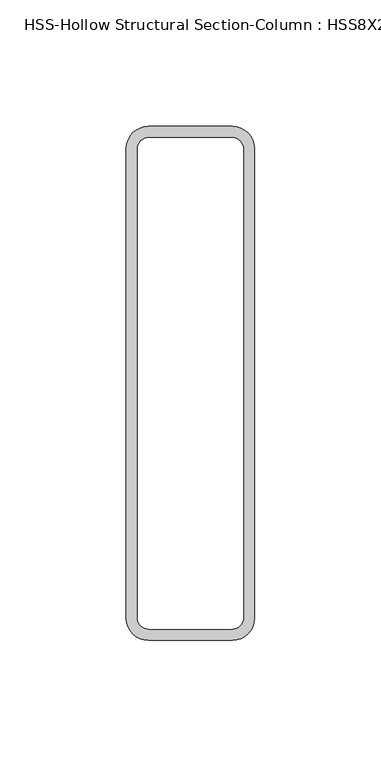
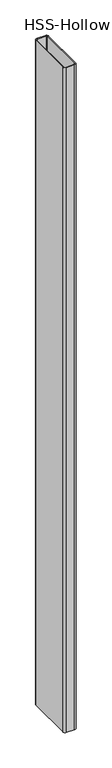
"""IFC4 building model written with IfcOpenShell, lengths in millimetres: column geometry, HSS-Hollow Structural Section-Column : HSS8X2X3/16."""

import ifcopenshell
import ifcopenshell.guid

model = None  # the IFC model being written
_history = None  # IfcOwnerHistory: only IFC2X3 demands one
_inside = {}  # id of a spatial element -> (the spatial element, [elements in it])
_under = {}  # id of a project, library or spatial element -> (it, [spatial elements below it])
_declared = {}  # id of a project -> (the project, [libraries it declares])
_typed = {}  # id of a type object -> (the type object, [elements of that type])
_made_of = {}  # id of a material, layer set ... -> (it, [elements and type objects made of it])


def new_model(schema):
    """Start an empty IFC model of exactly this schema.

    Asked for "IFC4X3", IfcOpenShell would pick the latest addendum, in which some entities
    have other attributes; the version numbers below select the first issue.
    IFC2X3 requires an IfcOwnerHistory on every rooted entity: one is made here for all.
    """
    global model, _history
    if schema == "IFC4X3":
        model = ifcopenshell.file(schema_version=(4, 3, 0, 0))
    else:
        model = ifcopenshell.file(schema=schema)
    _inside.clear()
    _under.clear()
    _declared.clear()
    _typed.clear()
    _made_of.clear()
    _history = None
    if model.schema == "IFC2X3":
        org = make("IfcOrganization", Name="unknown")
        user = make(
            "IfcPersonAndOrganization",
            ThePerson=make("IfcPerson", FamilyName="unknown"),
            TheOrganization=org,
        )
        app = make(
            "IfcApplication",
            ApplicationDeveloper=org,
            Version="unknown",
            ApplicationFullName="unknown",
            ApplicationIdentifier="unknown",
        )
        _history = make(
            "IfcOwnerHistory",
            OwningUser=user,
            OwningApplication=app,
            ChangeAction="ADDED",
            CreationDate=0,
        )
    return model


def make(cls, **values):
    """One entity of the class cls with the attributes given. An attribute that is None is left unset."""
    return model.create_entity(
        cls, **{name: value for name, value in values.items() if value is not None}
    )


def rooted(cls, **values):
    """An entity with a GlobalId (a new one), such as an element, a storey or a relation."""
    return make(cls, GlobalId=ifcopenshell.guid.new(), OwnerHistory=_history, **values)


def si_unit(unit_type, name, prefix=None):
    """IfcSIUnit, for example si_unit("LENGTHUNIT", "METRE", prefix="MILLI")."""
    return make("IfcSIUnit", UnitType=unit_type, Prefix=prefix, Name=name)


def assignment(units):
    """IfcUnitAssignment: the units of a project."""
    return None if units is None else make("IfcUnitAssignment", Units=units)


def point(xyz):
    """IfcCartesianPoint."""
    return None if xyz is None else make("IfcCartesianPoint", Coordinates=xyz)


def direction(xyz):
    """IfcDirection."""
    return None if xyz is None else make("IfcDirection", DirectionRatios=xyz)


def frame(location, z_axis=None, x_axis=None):
    """IfcAxis2Placement3D, a coordinate frame: its origin and axes. An axis left out is left unset."""
    return make(
        "IfcAxis2Placement3D",
        Location=point(location),
        Axis=direction(z_axis),
        RefDirection=direction(x_axis),
    )


def frame_2d(location, x_axis=None):
    """IfcAxis2Placement2D, a coordinate frame in the plane: its origin and x axis."""
    return make(
        "IfcAxis2Placement2D", Location=point(location), RefDirection=direction(x_axis)
    )


def origin():
    """The frame at (0, 0, 0) with its axes left unset."""
    return frame((0.0, 0.0, 0.0))


def place(relative_to, where):
    """IfcLocalPlacement: puts the frame where relative to a parent placement (None: the world)."""
    return make(
        "IfcLocalPlacement", PlacementRelTo=relative_to, RelativePlacement=where
    )


def context(
    kind, dimensions, precision=None, world=None, true_north=None, identifier=None
):
    """IfcGeometricRepresentationContext, for example the 3D "Model" context."""
    return make(
        "IfcGeometricRepresentationContext",
        ContextIdentifier=identifier,
        ContextType=kind,
        CoordinateSpaceDimension=dimensions,
        Precision=precision,
        WorldCoordinateSystem=world,
        TrueNorth=true_north,
    )


def project(units=None, contexts=None):
    """IfcProject with its units and contexts."""
    return rooted(
        "IfcProject",
        Name="project",
        RepresentationContexts=contexts,
        UnitsInContext=assignment(units),
    )


def spatial(cls, under=None, at=None, **own):
    """A site, building, storey or space (cls), placed at a placement, below another one or the project."""
    s = rooted(cls, ObjectPlacement=at, **own)
    if under is not None:
        _under.setdefault(under.id(), (under, []))[1].append(s)
    return s


def polyline(points):
    """IfcPolyline through the points."""
    return make("IfcPolyline", Points=[point(p) for p in points])


def circle_curve(where, radius):
    """IfcCircle in the frame where."""
    return make("IfcCircle", Position=where, Radius=radius)


def trimmed(basis, trim1, trim2, sense, master):
    """IfcTrimmedCurve: the piece of a basis curve between two trims."""
    return make(
        "IfcTrimmedCurve",
        BasisCurve=basis,
        Trim1=trim1,
        Trim2=trim2,
        SenseAgreement=sense,
        MasterRepresentation=master,
    )


def segment(curve, same_sense, transition):
    """IfcCompositeCurveSegment."""
    return make(
        "IfcCompositeCurveSegment",
        Transition=transition,
        SameSense=same_sense,
        ParentCurve=curve,
    )


def composite_curve(segments, self_intersect=None):
    """IfcCompositeCurve: segments joined end to end."""
    return make("IfcCompositeCurve", Segments=segments, SelfIntersect=self_intersect)


def outline(outer, holes=None, kind="AREA"):
    """IfcArbitraryClosedProfileDef: a profile drawn as a closed curve; with holes, ...WithVoids."""
    if holes is None:
        return make("IfcArbitraryClosedProfileDef", ProfileType=kind, OuterCurve=outer)
    return make(
        "IfcArbitraryProfileDefWithVoids",
        ProfileType=kind,
        OuterCurve=outer,
        InnerCurves=holes,
    )


def extrude(swept, where, along, depth):
    """IfcExtrudedAreaSolid: the profile swept, set in the frame where, extruded along a direction by depth."""
    return make(
        "IfcExtrudedAreaSolid",
        SweptArea=swept,
        Position=where,
        ExtrudedDirection=direction(along),
        Depth=depth,
    )


def shape(context_of_items, identifier, shape_type, items):
    """IfcShapeRepresentation: the items that make up one representation, for example the "Body"."""
    return make(
        "IfcShapeRepresentation",
        ContextOfItems=context_of_items,
        RepresentationIdentifier=identifier,
        RepresentationType=shape_type,
        Items=items,
    )


def source(mapping_origin, context_of_items, identifier, shape_type, items):
    """IfcRepresentationMap: a shape defined once, which mapped items show again and again."""
    return make(
        "IfcRepresentationMap",
        MappingOrigin=mapping_origin,
        MappedRepresentation=shape(context_of_items, identifier, shape_type, items),
    )


def transform(
    local_origin,
    x_axis=None,
    y_axis=None,
    z_axis=None,
    scale=None,
    scale2=None,
    scale3=None,
    uniform=True,
):
    """IfcCartesianTransformationOperator3D, or its non-uniform kind. x_axis, y_axis, z_axis: its Axis1, 2, 3."""
    if uniform:
        return make(
            "IfcCartesianTransformationOperator3D",
            Axis1=direction(x_axis),
            Axis2=direction(y_axis),
            LocalOrigin=point(local_origin),
            Scale=scale,
            Axis3=direction(z_axis),
        )
    return make(
        "IfcCartesianTransformationOperator3DnonUniform",
        Axis1=direction(x_axis),
        Axis2=direction(y_axis),
        LocalOrigin=point(local_origin),
        Scale=scale,
        Axis3=direction(z_axis),
        Scale2=scale2,
        Scale3=scale3,
    )


def mapped(mapping_source, mapping_target):
    """IfcMappedItem: shows the shape of a source again, moved by a transform."""
    return make(
        "IfcMappedItem", MappingSource=mapping_source, MappingTarget=mapping_target
    )


def made_of(thing, what):
    """Note that an element or type object is made of a material, layer set ...; save() writes the relation."""
    if what is not None:
        _made_of.setdefault(what.id(), (what, []))[1].append(thing)
    return thing


def element(
    cls,
    number,
    at=None,
    inside=None,
    cuts=None,
    type_object=None,
    material=None,
    context=None,
    identifier="Body",
    shape_type=None,
    held_by="IfcProductDefinitionShape",
    body=None,
    shapes=None,
    **own,
):
    """One element of the class cls, such as IfcWall. Its Tag is "e" and its number.

    at: its placement. inside: the storey or other place that contains it. cuts: it is an
    opening in that element (IfcRelVoidsElement). A single representation is given by context,
    identifier, shape_type and body (its items); several are given by shapes. held_by: the class
    of the entity that holds the representations. save() writes the other relations.
    """
    e = rooted(cls, Tag="e%d" % number, ObjectPlacement=at, **own)
    if body is not None:
        shapes = [shape(context, identifier, shape_type, body)]
    if shapes is not None:
        e.Representation = make(held_by, Representations=shapes)
    if inside is not None:
        _inside.setdefault(inside.id(), (inside, []))[1].append(e)
    if cuts is not None:
        rooted(
            "IfcRelVoidsElement", RelatingBuildingElement=cuts, RelatedOpeningElement=e
        )
    if type_object is not None:
        _typed.setdefault(type_object.id(), (type_object, []))[1].append(e)
    return made_of(e, material)


def aggregate(whole, parts):
    """IfcRelAggregates: a whole, such as a stair, and the parts it consists of."""
    return rooted("IfcRelAggregates", RelatingObject=whole, RelatedObjects=parts)


def save(model, path):
    """Write the relations noted so far, then the file.

    IfcRelAggregates (storeys below a building ...), IfcRelContainedInSpatialStructure (elements
    in a storey), IfcRelDefinesByType, IfcRelAssociatesMaterial and IfcRelDeclares: one each for
    every whole, place, type object, material and project.
    """
    for whole, parts in _under.values():
        aggregate(whole, parts)
    for where, things in _inside.values():
        rooted(
            "IfcRelContainedInSpatialStructure",
            RelatedElements=things,
            RelatingStructure=where,
        )
    for kind, things in _typed.values():
        rooted("IfcRelDefinesByType", RelatedObjects=things, RelatingType=kind)
    for what, things in _made_of.values():
        rooted("IfcRelAssociatesMaterial", RelatedObjects=things, RelatingMaterial=what)
    for by, libraries in _declared.values():
        rooted("IfcRelDeclares", RelatingContext=by, RelatedDefinitions=libraries)
    model.write(path)


def hss_hollow_structural_section_column_hss8x2x3_16_e82f30fd(model_context):
    return source(origin(), model_context, "Body", "SweptSolid", [
        extrude(outline(composite_curve([segment(trimmed(circle_curve(frame_2d((16.5608, 92.7608)), 8.8392), [point((16.5608, 101.6))], [point((25.4, 92.7608))], False, "CARTESIAN"), True, "CONTINUOUS"), segment(polyline([(25.4, 92.7608), (25.4, -92.7608)]), True, "CONTINUOUS"), segment(trimmed(circle_curve(frame_2d((16.5608, -92.7608)), 8.8392), [point((25.4, -92.7608))], [point((16.5608, -101.6))], False, "CARTESIAN"), True, "CONTINUOUS"), segment(polyline([(16.5608, -101.6), (-16.5608, -101.6)]), True, "CONTINUOUS"), segment(trimmed(circle_curve(frame_2d((-16.5608, -92.7608)), 8.8392), [point((-16.5608, -101.6))], [point((-25.4, -92.7608))], False, "CARTESIAN"), True, "CONTINUOUS"), segment(polyline([(-25.4, -92.7608), (-25.4, 92.7608)]), True, "CONTINUOUS"), segment(trimmed(circle_curve(frame_2d((-16.5608, 92.7608)), 8.8392), [point((-25.4, 92.7608))], [point((-16.5608, 101.6))], False, "CARTESIAN"), True, "CONTINUOUS"), segment(polyline([(-16.5608, 101.6), (16.5608, 101.6)]), True, "CONTINUOUS")], self_intersect=False), holes=[composite_curve([segment(polyline([(16.5608, 97.1804), (-16.5608, 97.1804)]), True, "CONTINUOUS"), segment(trimmed(circle_curve(frame_2d((-16.5608, 92.7608)), 4.4196), [point((-16.5608, 97.1804))], [point((-20.9804, 92.7608))], True, "CARTESIAN"), True, "CONTINUOUS"), segment(polyline([(-20.9804, 92.7608), (-20.9804, -92.7608)]), True, "CONTINUOUS"), segment(trimmed(circle_curve(frame_2d((-16.5608, -92.7608)), 4.4196), [point((-20.9804, -92.7608))], [point((-16.5608, -97.1804))], True, "CARTESIAN"), True, "CONTINUOUS"), segment(polyline([(-16.5608, -97.1804), (16.5608, -97.1804)]), True, "CONTINUOUS"), segment(trimmed(circle_curve(frame_2d((16.5608, -92.7608)), 4.4196), [point((16.5608, -97.1804))], [point((20.9804, -92.7608))], True, "CARTESIAN"), True, "CONTINUOUS"), segment(polyline([(20.9804, -92.7608), (20.9804, 92.7608)]), True, "CONTINUOUS"), segment(trimmed(circle_curve(frame_2d((16.5608, 92.7608)), 4.4196), [point((20.9804, 92.7608))], [point((16.5608, 97.1804))], True, "CARTESIAN"), True, "CONTINUOUS")], self_intersect=False)]), frame((0.0, 0.0, -594.0), z_axis=(0.0, 0.0, 1.0), x_axis=(1.0, 0.0, 0.0)), (0.0, 0.0, 1.0), 2793.0),
    ])


if __name__ == "__main__":
    model = new_model("IFC4")
    model_context = context("Model", 3, world=origin())
    ifc_project = project(units=[si_unit("LENGTHUNIT", "METRE", prefix="MILLI")], contexts=[model_context])
    site = spatial("IfcSite", under=ifc_project)
    building = spatial("IfcBuilding", under=site)
    placement = place(None, origin())
    hss_hollow_structural_section_column_hss8x2x3_16_shape = hss_hollow_structural_section_column_hss8x2x3_16_e82f30fd(model_context)
    element("IfcColumn", 1, ObjectType="HSS-Hollow Structural Section-Column : HSS8X2X3/16", at=placement, inside=building, context=model_context, shape_type="MappedRepresentation", body=[
        mapped(hss_hollow_structural_section_column_hss8x2x3_16_shape, transform((0.0, 0.0, 0.0), x_axis=(1.0, 0.0, 0.0), y_axis=(0.0, 1.0, 0.0), z_axis=(0.0, 0.0, 1.0))),
    ])
    save(model, "model.ifc")

# Revit data of these elements
# Type "HSS-Hollow Structural Section-Column : HSS8X2X3/16"
#   Assembly Code = "B10"
#   Shape = "Rect."
#   Cost = 1
#   W = 12
#   Ht = 203.2 mm
#   b = 50.8 mm
#   kr = 8.839 mm
#   t = 4.42 mm
#   A = 0.00211612 m²
#   Structural Material [instance default] = Steel ASTM A500, Grade B, Rectangular and Square
# Element 1 (IfcColumn, "HSS-Hollow Structural Section-Column : HSS8X2X3/16")
#   Structural Material = Metal - Steel 43-275
#   Materials on its faces: "Metal - Steel 43-275"
# Materials
#   "Steel ASTM A500, Grade B, Rectangular and Square": class "Metal", colour RGB 199 199 199, transparency 0, Description = "Carbon steel", Cost = 0
#   "Metal - Steel 43-275": class "Metal", colour RGB 247 247 247, transparency 0, Cost = 0
